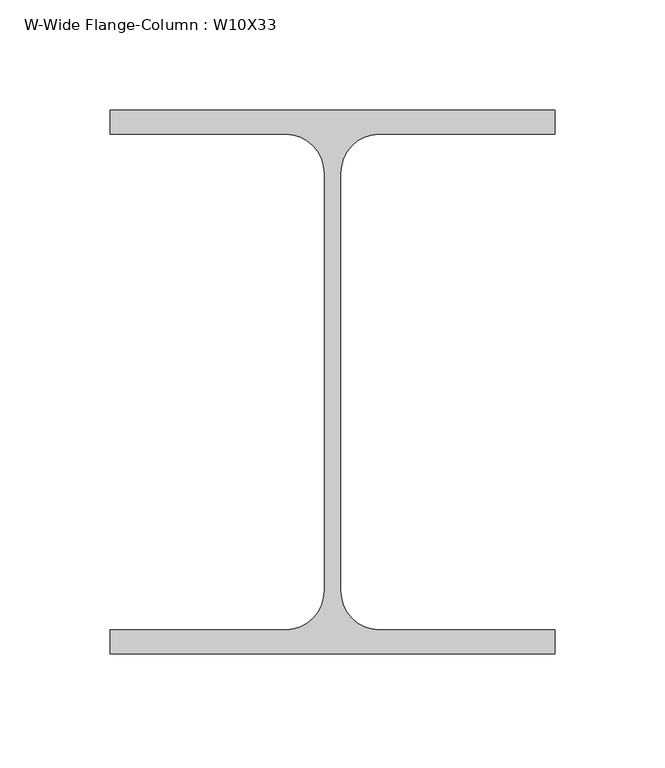
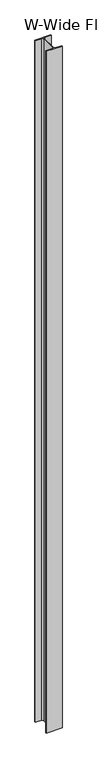
"""IFC4 building model written with IfcOpenShell, lengths in millimetres: column geometry, W-Wide Flange-Column : W10X33."""

from ifc_helpers import new_model, si_unit, point, frame, frame_2d, origin, place, context, project, spatial, polyline, circle_curve, trimmed, segment, composite_curve, outline, extrude, source, transform, mapped, element, save


def w_wide_flange_column_w10x33_beb9aee9(model_context):
    return source(origin(), model_context, "Body", "SweptSolid", [
        extrude(outline(composite_curve([segment(polyline([(101.092, 123.571), (101.092, 112.522), (21.209, 112.522)]), True, "CONTINUOUS"), segment(trimmed(circle_curve(frame_2d((21.209, 94.996)), 17.526), [point((21.209, 112.522))], [point((3.683, 94.996))], True, "CARTESIAN"), True, "CONTINUOUS"), segment(polyline([(3.683, 94.996), (3.683, -94.996)]), True, "CONTINUOUS"), segment(trimmed(circle_curve(frame_2d((21.209, -94.996)), 17.526), [point((3.683, -94.996))], [point((21.209, -112.522))], True, "CARTESIAN"), True, "CONTINUOUS"), segment(polyline([(21.209, -112.522), (101.092, -112.522), (101.092, -123.571), (-101.092, -123.571), (-101.092, -112.522), (-21.209, -112.522)]), True, "CONTINUOUS"), segment(trimmed(circle_curve(frame_2d((-21.209, -94.996)), 17.526), [point((-21.209, -112.522))], [point((-3.683, -94.996))], True, "CARTESIAN"), True, "CONTINUOUS"), segment(polyline([(-3.683, -94.996), (-3.683, 94.996)]), True, "CONTINUOUS"), segment(trimmed(circle_curve(frame_2d((-21.209, 94.996)), 17.526), [point((-3.683, 94.996))], [point((-21.209, 112.522))], True, "CARTESIAN"), True, "CONTINUOUS"), segment(polyline([(-21.209, 112.522), (-101.092, 112.522), (-101.092, 123.571), (101.092, 123.571)]), True, "CONTINUOUS")], self_intersect=False)), frame((0.0, 0.0, 12725.4), z_axis=(0.0, 0.0, 1.0), x_axis=(1.0, 0.0, 0.0)), (0.0, 0.0, 1.0), 9169.4),
    ])


if __name__ == "__main__":
    model = new_model("IFC4")
    model_context = context("Model", 3, world=origin())
    ifc_project = project(units=[si_unit("LENGTHUNIT", "METRE", prefix="MILLI")], contexts=[model_context])
    site = spatial("IfcSite", under=ifc_project)
    building = spatial("IfcBuilding", under=site)
    placement = place(None, origin())
    w_wide_flange_column_w10x33_shape = w_wide_flange_column_w10x33_beb9aee9(model_context)
    element("IfcColumn", 1, ObjectType="W-Wide Flange-Column : W10X33", at=placement, inside=building, context=model_context, shape_type="MappedRepresentation", body=[
        mapped(w_wide_flange_column_w10x33_shape, transform((0.0, 0.0, 0.0), x_axis=(1.0, 0.0, 0.0), y_axis=(0.0, 1.0, 0.0), z_axis=(0.0, 0.0, 1.0))),
    ])
    save(model, "model.ifc")

# Revit data of these elements
# Type "W-Wide Flange-Column : W10X33"
#   Assembly Code = "B10"
#   W = 33
#   bf = 0' - 7.96"
#   d = 0' - 9.73"
#   k = 0' - 1 1/8"
#   kr = 0' - 0.69"
#   tf = 0' - 0.435"
#   tw = 0' - 0.29"
#   A = 0.0674306 SF
#   Structural Material [instance default] = Steel ASTM A992
# Element 1 (IfcColumn, "W-Wide Flange-Column : W10X33")
#   Materials on its faces: "Steel ASTM A992"
# Materials
#   "Steel ASTM A992": class "Metal", colour RGB 199 199 199, transparency 0, Description = "Structural steel 50ksi", Cost = 0
